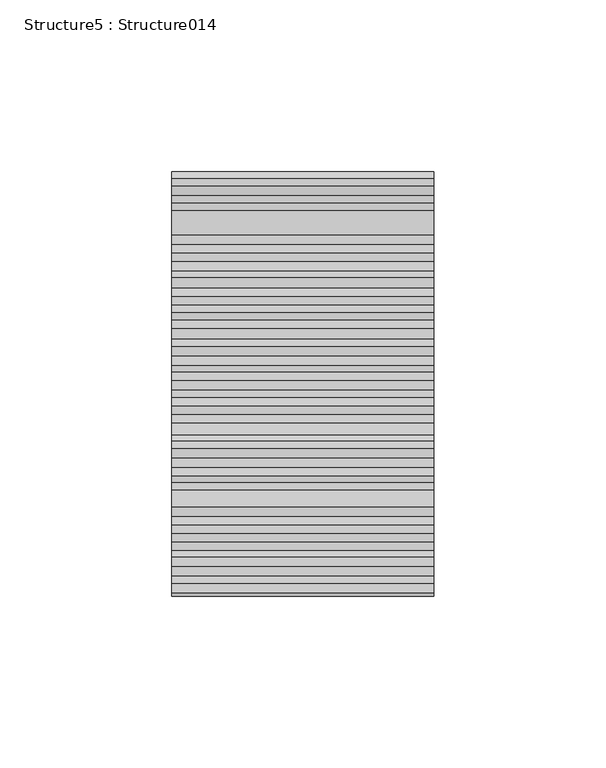
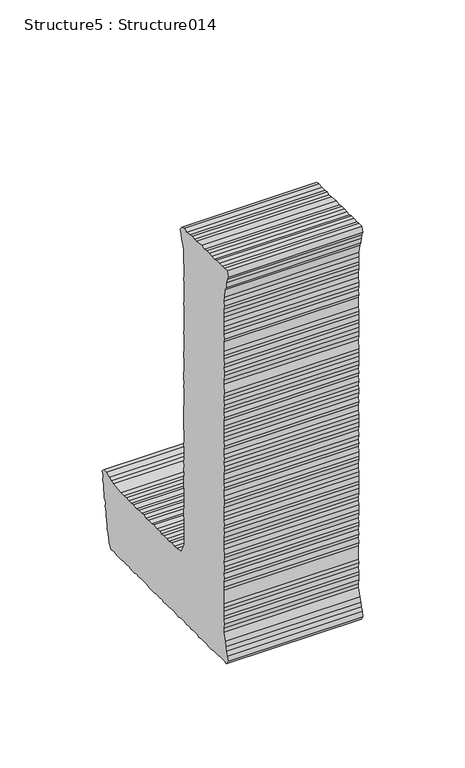
"""IFC4 building model written with IfcOpenShell, lengths in millimetres: proxy geometry, Structure5 : Structure014."""

from ifc_helpers import new_model, si_unit, frame, origin, place, context, project, spatial, polyline, outline, extrude, source, transform, mapped, element, save


def structure5_structure014_57d267da(model_context):
    return source(origin(), model_context, "Body", "SweptSolid", [
        extrude(outline(polyline([(2.6214432, 0.0), (3.4974043, -2.2001182), (5.9028767, -4.170302), (6.5519255, -6.1432533), (8.2949405, -7.8974569), (10.0261775, -10.5244387), (11.5590037, -12.0671042), (11.9767249, -14.2567705), (13.9510714, -15.793061), (15.267169, -18.4193137), (16.7862613, -19.9481571), (18.3073094, -22.3636009), (19.3900622, -24.3391377), (21.1330772, -26.0933413), (22.0060526, -28.2904546), (23.5321209, -30.2602212), (25.2731015, -32.4631068), (25.7022466, -35.9503522), (23.066859, -37.6875528), (21.9630707, -39.6656792), (19.776365, -41.4049143), (18.674615, -42.9331606), (16.4809333, -44.2314725), (14.9524555, -46.1980563), (12.7501708, -47.9384398), (11.4378493, -50.1237693), (9.4600884, -52.0889158), (7.7003001, -52.9561017), (6.1718223, -54.9226855), (4.4104072, -56.6728661), (2.6588429, -57.9654038), (0.8980288, -59.7149873), (-0.8565997, -62.3398027), (-4.3620021, -65.8228471), (-6.338737, -66.905596), (-7.8764187, -69.3148484), (-9.8539902, -70.8462832), (-10.9479277, -72.3667669), (-13.1340324, -74.1054048), (-14.2447967, -75.642608), (-16.4315023, -77.3818431), (-18.4162393, -78.9060664), (-19.7285608, -81.091396), (-21.2556014, -82.6086969), (-23.4576966, -83.9153686), (-25.2106982, -85.6571893), (-26.7561924, -88.0742044), (-29.1668209, -89.5880793), (-30.2535928, -91.1157745), (-32.4552765, -92.8555607), (-34.4336383, -94.8213043), (-35.303052, -96.566551), (-37.2812244, -98.0985829), (-39.2511727, -100.0559666), (-41.0105495, -101.3562671), (-42.1059243, -103.3260337), (-43.8667385, -105.0756172), (-46.5027271, -106.8134148), (-53.5225462, -113.7884606), (-54.6171306, -115.3239184), (-57.450908, -114.6594917), (-58.9827543, -112.2488056), (-59.8491613, -110.0583029), (-61.1564378, -107.858003), (-62.6793311, -105.4575295), (-64.8530146, -101.0667269), (-66.3721068, -99.5378835), (-68.7729381, -97.9894457), (-70.5271628, -95.8068854), (-71.8294977, -94.4961908), (-73.5806294, -92.2830889), (-75.5454218, -90.7564138), (-76.839751, -89.0030467), (-82.5124618, -83.2939224), (-84.0461282, -82.2011408), (-86.0014775, -79.7825104), (-87.9640172, -78.6751777), (-89.4934789, -76.2680937), (-91.6703873, -74.9450161), (-92.9792907, -73.6277108), (-94.2884122, -71.4423813), (-96.8958496, -69.6860112), (-98.214307, -68.3590905), (-100.176332, -65.967396), (-101.6939869, -63.9892697), (-103.0028902, -62.6719644), (-104.9712654, -61.1416836), (-107.369465, -59.1451648), (-108.6871895, -57.4019066), (-110.4213834, -56.073656), (-112.3929624, -53.6723461), (-113.9186231, -52.1368921), (-115.2195208, -50.3769144), (-117.179293, -48.4045622), (-119.5765415, -46.8597302), (-120.8884305, -45.5394201), (-122.4199266, -43.5810181), (-124.3776644, -41.159984), (-126.3378156, -40.055055), (-127.4295828, -38.0884751), (-129.4045263, -36.5515837), (-131.3527102, -34.1401649), (-133.5260358, -32.8206931), (-135.2756192, -31.0598789), (-136.5933438, -29.3166208), (-138.5442949, -27.7702214), (-139.6360621, -25.8036415), (-141.8167716, -23.6089339), (-143.7864768, -22.4943896), (-145.3087729, -20.0945171), (-147.2777452, -18.5636354), (-149.0267315, -16.8034222), (-150.1037063, -15.2688047), (-152.0786499, -13.7319133), (-154.0339992, -11.313283), (-155.9869848, -10.2155656), (-157.3020777, -8.0242264), (-159.0536956, -6.7120942), (-161.2184184, -4.950551), (-162.7600657, -2.9819327), (-164.2851292, -1.4470797), (-166.2432459, 0.1065312), (-169.2953825, 4.0460643), (-171.2697289, 5.5823547), (-173.6488206, 7.5596428), (-175.1744811, 9.0950967), (-176.7191141, 11.0667198), (-178.4437539, 12.3853552), (-180.4159301, 14.787266), (-181.7278191, 16.1075762), (-183.2412941, 18.0814957), (-187.1745726, 22.0400222), (-188.9113981, 22.920192), (-190.4438454, 25.3302807), (-192.1948662, 26.6418119), (-193.9438525, 28.4020251), (-195.675279, 30.5952953), (-197.6422169, 32.574859), (-199.6165633, 34.1111494), (-201.3565926, 35.8623482), (-202.8674609, 36.9658397), (-204.6252683, 39.1520057), (-206.7899911, 40.913549), (-210.5081392, 43.7709322), (-212.9124424, 44.4214049), (-215.3095014, 46.3999486), (-217.4923812, 47.7290357), (-219.4545707, 48.3840845), (-220.9849796, 51.2440534), (-219.0072187, 53.2091999), (-217.2658056, 54.511954), (-215.5012155, 56.6928414), (-213.5234546, 58.6579878), (-211.7720798, 59.516814), (-210.2465875, 61.4864026), (-208.698944, 63.451727), (-206.9459424, 65.1935478), (-204.7444482, 66.4996224), (-203.2151799, 68.900515), (-199.2606841, 71.9484104), (-197.7246292, 73.4746681), (-196.8468019, 75.2282746), (-194.6531203, 76.5265865), (-192.6747584, 78.4923301), (-191.1460911, 80.8926255), (-189.1693562, 81.9753745), (-186.542135, 81.5344551), (-185.4613592, 79.1282076), (-183.9373254, 76.7097589), (-182.8533745, 74.7342183), (-181.5486262, 72.1181857), (-178.2729744, 68.387605), (-176.7473137, 66.852151), (-175.0063332, 64.6492654), (-171.2999632, 60.9191039), (-169.7656996, 59.8257214), (-168.0344626, 57.1987395), (-164.7592185, 53.9024714), (-162.7992568, 52.3638309), (-161.0498628, 50.169305), (-159.0812982, 49.072736), (-157.7847699, 46.8832533), (-155.817235, 44.9030886), (-153.8578704, 43.365049), (-150.3688547, 39.853637), (-148.8427864, 37.8838705), (-146.6508961, 36.5625422), (-145.7914651, 34.8129626), (-142.2988667, 31.2979449), (-140.3418906, 29.7623091), (-137.9328353, 27.7885196), (-134.8831409, 23.834617), (-133.3568831, 22.2985621), (-131.4011013, 20.7641282), (-129.6494833, 19.4519961), (-127.6831426, 17.4730333), (-126.1680657, 15.0635991), (-124.4078985, 14.1767652), (-122.6764721, 11.983495), (-120.9340542, 10.2298924), (-119.1846602, 8.0353666), (-117.4446308, 6.2841679), (-115.2587118, 4.9688492), (-106.7586026, -3.5858229), (-105.2343793, -5.5705599), (-103.2712137, -7.9802295), (-101.751932, -9.0753613), (-99.7769884, -10.6122526), (-98.2529546, -13.0307011), (-96.2929929, -14.5693417), (-94.3296379, -16.5452997), (-92.3612626, -18.0755804), (-91.0609622, -19.8349572), (-89.3099413, -21.1464883), (-87.3545921, -23.5651188), (-85.3802456, -25.1014091), (-81.9037696, -28.6002009), (-81.0276191, -30.3666074), (-79.0676574, -31.9052479), (-73.8356267, -37.1708634), (-71.6439258, -38.9259034), (-70.1278192, -40.451742), (-68.3870281, -43.0883392), (-66.861178, -44.1900816), (-63.1452539, -47.9298584), (-61.846094, -49.67126), (-59.6623989, -51.8689724), (-57.9197916, -53.1888634), (-53.7661194, -54.7309279), (-51.8039337, -55.3871749), (-47.8514723, -52.7879614), (-45.8817135, -51.2642894), (-44.5615794, -49.071197), (-42.3678977, -47.7728852), (-40.8234293, -46.2382676), (-39.0708392, -44.0633323), (-37.1010802, -42.5396602), (-35.9993302, -41.0114139), (-33.8042112, -39.263819), (-32.2749429, -36.8629264), (-30.2988088, -35.7807745), (-28.3202576, -33.3813194), (-26.3504987, -31.8576472), (-25.2473113, -29.880118), (-23.4957471, -28.5875802), (-21.9582548, -26.6120394), (-19.765174, -25.3143246), (-18.0105455, -22.6895092), (-16.4681155, -21.6047718), (-14.2814099, -19.8655367), (-12.7451655, -17.9055672), (-10.7675941, -16.3741325), (-9.0059896, -14.1902403), (-4.628538, -8.51267), (-3.5157967, -6.5447562), (-2.4288351, -4.5833494), (-1.3102833, -1.7354495), (0.0, 0.0), (2.6214432, 0.0)])), frame((-35624.0862846, 276844.2032848, 4026.1308942), z_axis=(1.0, 0.0, 1.354250045437766e-12), x_axis=(0.0, 0.7093653755275494, -0.7048409494365795)), (0.0, 0.0, 1.0), 76.2),
    ])


if __name__ == "__main__":
    model = new_model("IFC4")
    model_context = context("Model", 3, world=origin())
    ifc_project = project(units=[si_unit("LENGTHUNIT", "METRE", prefix="MILLI")], contexts=[model_context])
    site = spatial("IfcSite", under=ifc_project)
    building = spatial("IfcBuilding", under=site)
    placement = place(None, origin())
    structure5_structure014_shape = structure5_structure014_57d267da(model_context)
    element("IfcBuildingElementProxy", 1, Name="Structure5 : Structure014", ObjectType="Structure5 : Structure014", at=placement, inside=building, context=model_context, shape_type="MappedRepresentation", body=[
        mapped(structure5_structure014_shape, transform((0.0, 0.0, 0.0), x_axis=(1.0, 0.0, 0.0), y_axis=(0.0, 1.0, 0.0), z_axis=(0.0, 0.0, 1.0))),
    ])
    save(model, "model.ifc")

# Revit data of these elements
# Type "Structure5 : Structure014"
#   NameOverride = "Structure014"
# Element 1 (IfcBuildingElementProxy, "Structure5 : Structure014")
#   Materials on its faces: "BRUSHED ALUMINUM LETTERING"
# Materials
#   "BRUSHED ALUMINUM LETTERING": class "Unassigned", colour RGB 169 181 186, transparency 0, Cost = 0
